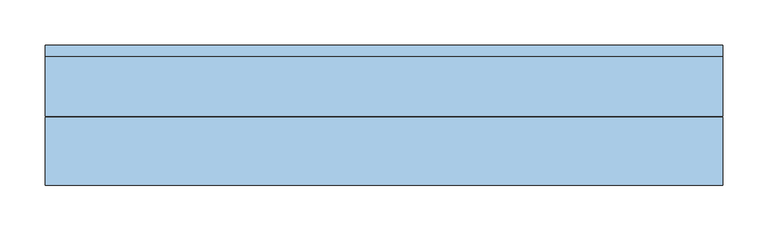
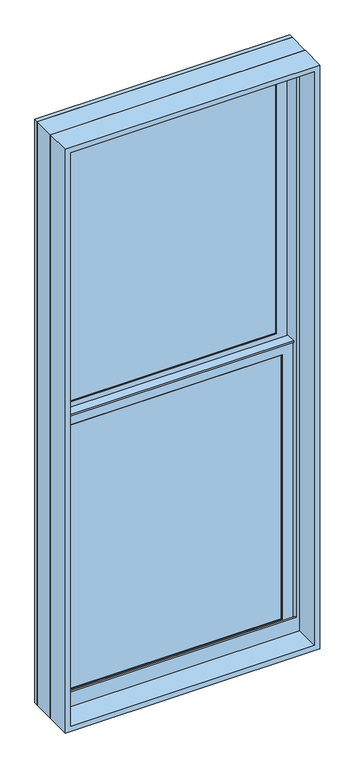
"""IFC4 building model written with IfcOpenShell, lengths in millimetres: window geometry, Window-Double_Hung-Marvin-Essential : ESDH2660."""

import ifcopenshell
import ifcopenshell.guid

model = None  # the IFC model being written
_history = None  # IfcOwnerHistory: only IFC2X3 demands one
_inside = {}  # id of a spatial element -> (the spatial element, [elements in it])
_under = {}  # id of a project, library or spatial element -> (it, [spatial elements below it])
_declared = {}  # id of a project -> (the project, [libraries it declares])
_typed = {}  # id of a type object -> (the type object, [elements of that type])
_made_of = {}  # id of a material, layer set ... -> (it, [elements and type objects made of it])


def new_model(schema):
    """Start an empty IFC model of exactly this schema.

    Asked for "IFC4X3", IfcOpenShell would pick the latest addendum, in which some entities
    have other attributes; the version numbers below select the first issue.
    IFC2X3 requires an IfcOwnerHistory on every rooted entity: one is made here for all.
    """
    global model, _history
    if schema == "IFC4X3":
        model = ifcopenshell.file(schema_version=(4, 3, 0, 0))
    else:
        model = ifcopenshell.file(schema=schema)
    _inside.clear()
    _under.clear()
    _declared.clear()
    _typed.clear()
    _made_of.clear()
    _history = None
    if model.schema == "IFC2X3":
        org = make("IfcOrganization", Name="unknown")
        user = make(
            "IfcPersonAndOrganization",
            ThePerson=make("IfcPerson", FamilyName="unknown"),
            TheOrganization=org,
        )
        app = make(
            "IfcApplication",
            ApplicationDeveloper=org,
            Version="unknown",
            ApplicationFullName="unknown",
            ApplicationIdentifier="unknown",
        )
        _history = make(
            "IfcOwnerHistory",
            OwningUser=user,
            OwningApplication=app,
            ChangeAction="ADDED",
            CreationDate=0,
        )
    return model


def make(cls, **values):
    """One entity of the class cls with the attributes given. An attribute that is None is left unset."""
    return model.create_entity(
        cls, **{name: value for name, value in values.items() if value is not None}
    )


def rooted(cls, **values):
    """An entity with a GlobalId (a new one), such as an element, a storey or a relation."""
    return make(cls, GlobalId=ifcopenshell.guid.new(), OwnerHistory=_history, **values)


def si_unit(unit_type, name, prefix=None):
    """IfcSIUnit, for example si_unit("LENGTHUNIT", "METRE", prefix="MILLI")."""
    return make("IfcSIUnit", UnitType=unit_type, Prefix=prefix, Name=name)


def assignment(units):
    """IfcUnitAssignment: the units of a project."""
    return None if units is None else make("IfcUnitAssignment", Units=units)


def point(xyz):
    """IfcCartesianPoint."""
    return None if xyz is None else make("IfcCartesianPoint", Coordinates=xyz)


def direction(xyz):
    """IfcDirection."""
    return None if xyz is None else make("IfcDirection", DirectionRatios=xyz)


def frame(location, z_axis=None, x_axis=None):
    """IfcAxis2Placement3D, a coordinate frame: its origin and axes. An axis left out is left unset."""
    return make(
        "IfcAxis2Placement3D",
        Location=point(location),
        Axis=direction(z_axis),
        RefDirection=direction(x_axis),
    )


def origin():
    """The frame at (0, 0, 0) with its axes left unset."""
    return frame((0.0, 0.0, 0.0))


def place(relative_to, where):
    """IfcLocalPlacement: puts the frame where relative to a parent placement (None: the world)."""
    return make(
        "IfcLocalPlacement", PlacementRelTo=relative_to, RelativePlacement=where
    )


def context(
    kind, dimensions, precision=None, world=None, true_north=None, identifier=None
):
    """IfcGeometricRepresentationContext, for example the 3D "Model" context."""
    return make(
        "IfcGeometricRepresentationContext",
        ContextIdentifier=identifier,
        ContextType=kind,
        CoordinateSpaceDimension=dimensions,
        Precision=precision,
        WorldCoordinateSystem=world,
        TrueNorth=true_north,
    )


def project(units=None, contexts=None):
    """IfcProject with its units and contexts."""
    return rooted(
        "IfcProject",
        Name="project",
        RepresentationContexts=contexts,
        UnitsInContext=assignment(units),
    )


def spatial(cls, under=None, at=None, **own):
    """A site, building, storey or space (cls), placed at a placement, below another one or the project."""
    s = rooted(cls, ObjectPlacement=at, **own)
    if under is not None:
        _under.setdefault(under.id(), (under, []))[1].append(s)
    return s


def polyline(points):
    """IfcPolyline through the points."""
    return make("IfcPolyline", Points=[point(p) for p in points])


def outline(outer, holes=None, kind="AREA"):
    """IfcArbitraryClosedProfileDef: a profile drawn as a closed curve; with holes, ...WithVoids."""
    if holes is None:
        return make("IfcArbitraryClosedProfileDef", ProfileType=kind, OuterCurve=outer)
    return make(
        "IfcArbitraryProfileDefWithVoids",
        ProfileType=kind,
        OuterCurve=outer,
        InnerCurves=holes,
    )


def extrude(swept, where, along, depth):
    """IfcExtrudedAreaSolid: the profile swept, set in the frame where, extruded along a direction by depth."""
    return make(
        "IfcExtrudedAreaSolid",
        SweptArea=swept,
        Position=where,
        ExtrudedDirection=direction(along),
        Depth=depth,
    )


def faces_of(points, faces, orient=None, outer=None):
    """IfcFace entities. A face is a list of loops; a loop is a list of indices into points, from 0.

    orient and outer hold one flag for each loop. By default every Orientation is true, the
    first loop of a face is its IfcFaceOuterBound and the others are IfcFaceBound.
    """
    made = []
    for i, loops in enumerate(faces):
        bounds = []
        for j, loop in enumerate(loops):
            is_outer = j == 0 if outer is None else outer[i][j]
            bounds.append(
                make(
                    "IfcFaceOuterBound" if is_outer else "IfcFaceBound",
                    Bound=make("IfcPolyLoop", Polygon=[points[k] for k in loop]),
                    Orientation=True if orient is None else orient[i][j],
                )
            )
        made.append(make("IfcFace", Bounds=bounds))
    return made


def faceted_brep(points, faces, orient=None, outer=None, voids=None):
    """IfcFacetedBrep: a solid bounded by flat faces; with voids (closed shells), ...WithVoids."""
    shared = [point(p) for p in points]
    hull = make("IfcClosedShell", CfsFaces=faces_of(shared, faces, orient, outer))
    if voids is None:
        return make("IfcFacetedBrep", Outer=hull)
    return make(
        "IfcFacetedBrepWithVoids",
        Outer=hull,
        Voids=[
            make(cls, CfsFaces=faces_of(shared, fs, o, b)) for cls, fs, o, b in voids
        ],
    )


def shape(context_of_items, identifier, shape_type, items):
    """IfcShapeRepresentation: the items that make up one representation, for example the "Body"."""
    return make(
        "IfcShapeRepresentation",
        ContextOfItems=context_of_items,
        RepresentationIdentifier=identifier,
        RepresentationType=shape_type,
        Items=items,
    )


def source(mapping_origin, context_of_items, identifier, shape_type, items):
    """IfcRepresentationMap: a shape defined once, which mapped items show again and again."""
    return make(
        "IfcRepresentationMap",
        MappingOrigin=mapping_origin,
        MappedRepresentation=shape(context_of_items, identifier, shape_type, items),
    )


def transform(
    local_origin,
    x_axis=None,
    y_axis=None,
    z_axis=None,
    scale=None,
    scale2=None,
    scale3=None,
    uniform=True,
):
    """IfcCartesianTransformationOperator3D, or its non-uniform kind. x_axis, y_axis, z_axis: its Axis1, 2, 3."""
    if uniform:
        return make(
            "IfcCartesianTransformationOperator3D",
            Axis1=direction(x_axis),
            Axis2=direction(y_axis),
            LocalOrigin=point(local_origin),
            Scale=scale,
            Axis3=direction(z_axis),
        )
    return make(
        "IfcCartesianTransformationOperator3DnonUniform",
        Axis1=direction(x_axis),
        Axis2=direction(y_axis),
        LocalOrigin=point(local_origin),
        Scale=scale,
        Axis3=direction(z_axis),
        Scale2=scale2,
        Scale3=scale3,
    )


def mapped(mapping_source, mapping_target):
    """IfcMappedItem: shows the shape of a source again, moved by a transform."""
    return make(
        "IfcMappedItem", MappingSource=mapping_source, MappingTarget=mapping_target
    )


def made_of(thing, what):
    """Note that an element or type object is made of a material, layer set ...; save() writes the relation."""
    if what is not None:
        _made_of.setdefault(what.id(), (what, []))[1].append(thing)
    return thing


def element(
    cls,
    number,
    at=None,
    inside=None,
    cuts=None,
    type_object=None,
    material=None,
    context=None,
    identifier="Body",
    shape_type=None,
    held_by="IfcProductDefinitionShape",
    body=None,
    shapes=None,
    **own,
):
    """One element of the class cls, such as IfcWall. Its Tag is "e" and its number.

    at: its placement. inside: the storey or other place that contains it. cuts: it is an
    opening in that element (IfcRelVoidsElement). A single representation is given by context,
    identifier, shape_type and body (its items); several are given by shapes. held_by: the class
    of the entity that holds the representations. save() writes the other relations.
    """
    e = rooted(cls, Tag="e%d" % number, ObjectPlacement=at, **own)
    if body is not None:
        shapes = [shape(context, identifier, shape_type, body)]
    if shapes is not None:
        e.Representation = make(held_by, Representations=shapes)
    if inside is not None:
        _inside.setdefault(inside.id(), (inside, []))[1].append(e)
    if cuts is not None:
        rooted(
            "IfcRelVoidsElement", RelatingBuildingElement=cuts, RelatedOpeningElement=e
        )
    if type_object is not None:
        _typed.setdefault(type_object.id(), (type_object, []))[1].append(e)
    return made_of(e, material)


def aggregate(whole, parts):
    """IfcRelAggregates: a whole, such as a stair, and the parts it consists of."""
    return rooted("IfcRelAggregates", RelatingObject=whole, RelatedObjects=parts)


def save(model, path):
    """Write the relations noted so far, then the file.

    IfcRelAggregates (storeys below a building ...), IfcRelContainedInSpatialStructure (elements
    in a storey), IfcRelDefinesByType, IfcRelAssociatesMaterial and IfcRelDeclares: one each for
    every whole, place, type object, material and project.
    """
    for whole, parts in _under.values():
        aggregate(whole, parts)
    for where, things in _inside.values():
        rooted(
            "IfcRelContainedInSpatialStructure",
            RelatedElements=things,
            RelatingStructure=where,
        )
    for kind, things in _typed.values():
        rooted("IfcRelDefinesByType", RelatedObjects=things, RelatingType=kind)
    for what, things in _made_of.values():
        rooted("IfcRelAssociatesMaterial", RelatedObjects=things, RelatingMaterial=what)
    for by, libraries in _declared.values():
        rooted("IfcRelDeclares", RelatingContext=by, RelatedDefinitions=libraries)
    model.write(path)


def window_e5f0666e(model_context):
    return source(origin(), model_context, "Body", "SolidModel", [
        extrude(outline(polyline([(115.3583333, 20.6375), (115.3583333, 15.875), (96.3083333, 15.875), (96.3083333, 20.6375), (115.3583333, 20.6375)])), frame((0.0, 0.0, 679.45), z_axis=(0.0, 0.0, 1.0), x_axis=(1.0, 0.0, 0.0)), (0.0, 0.0, 1.0), 831.85),
        extrude(outline(polyline([(-96.3083333, 20.6375), (-96.3083333, 15.875), (-115.3583333, 15.875), (-115.3583333, 20.6375), (-96.3083333, 20.6375)])), frame((0.0, 0.0, 679.45), z_axis=(0.0, 0.0, 1.0), x_axis=(1.0, 0.0, 0.0)), (0.0, 0.0, 1.0), 831.85),
        extrude(outline(polyline([(317.5, 20.6375), (317.5, 15.875), (-317.5, 15.875), (-317.5, 20.6375), (317.5, 20.6375)])), frame((0.0, 0.0, 1085.85), z_axis=(0.0, 0.0, 1.0), x_axis=(1.0, 0.0, 0.0)), (0.0, 0.0, 1.0), 19.05),
        extrude(outline(polyline([(-115.3583333, 46.83125), (-115.3583333, 51.59375), (-96.3083333, 51.59375), (-96.3083333, 46.83125), (-115.3583333, 46.83125)])), frame((0.0, 0.0, 1549.4), z_axis=(0.0, 0.0, 1.0), x_axis=(1.0, 0.0, 0.0)), (0.0, 0.0, 1.0), 831.85),
        extrude(outline(polyline([(96.3083333, 46.83125), (96.3083333, 51.59375), (115.3583333, 51.59375), (115.3583333, 46.83125), (96.3083333, 46.83125)])), frame((0.0, 0.0, 1549.4), z_axis=(0.0, 0.0, 1.0), x_axis=(1.0, 0.0, 0.0)), (0.0, 0.0, 1.0), 831.85),
        extrude(outline(polyline([(-317.5, 46.83125), (-317.5, 51.59375), (317.5, 51.59375), (317.5, 46.83125), (-317.5, 46.83125)])), frame((0.0, 0.0, 1955.8), z_axis=(0.0, 0.0, 1.0), x_axis=(1.0, 0.0, 0.0)), (0.0, 0.0, 1.0), 19.05),
        extrude(outline(polyline([(115.3583333, 20.6375), (96.3083333, 20.6375), (96.3083333, 25.4), (115.3583333, 25.4), (115.3583333, 20.6375)])), frame((0.0, 0.0, 679.45), z_axis=(0.0, 0.0, 1.0), x_axis=(1.0, 0.0, 0.0)), (0.0, 0.0, 1.0), 831.85),
        extrude(outline(polyline([(-96.3083333, 20.6375), (-115.3583333, 20.6375), (-115.3583333, 25.4), (-96.3083333, 25.4), (-96.3083333, 20.6375)])), frame((0.0, 0.0, 679.45), z_axis=(0.0, 0.0, 1.0), x_axis=(1.0, 0.0, 0.0)), (0.0, 0.0, 1.0), 831.85),
        extrude(outline(polyline([(317.5, 20.6375), (-317.5, 20.6375), (-317.5, 25.4), (317.5, 25.4), (317.5, 20.6375)])), frame((0.0, 0.0, 1085.85), z_axis=(0.0, 0.0, 1.0), x_axis=(1.0, 0.0, 0.0)), (0.0, 0.0, 1.0), 19.05),
        extrude(outline(polyline([(-115.3583333, 56.35625), (-96.3083333, 56.35625), (-96.3083333, 51.59375), (-115.3583333, 51.59375), (-115.3583333, 56.35625)])), frame((0.0, 0.0, 1549.4), z_axis=(0.0, 0.0, 1.0), x_axis=(1.0, 0.0, 0.0)), (0.0, 0.0, 1.0), 831.85),
        extrude(outline(polyline([(96.3083333, 56.35625), (115.3583333, 56.35625), (115.3583333, 51.59375), (96.3083333, 51.59375), (96.3083333, 56.35625)])), frame((0.0, 0.0, 1549.4), z_axis=(0.0, 0.0, 1.0), x_axis=(1.0, 0.0, 0.0)), (0.0, 0.0, 1.0), 831.85),
        extrude(outline(polyline([(-317.5, 56.35625), (317.5, 56.35625), (317.5, 51.59375), (-317.5, 51.59375), (-317.5, 56.35625)])), frame((0.0, 0.0, 1955.8), z_axis=(0.0, 0.0, 1.0), x_axis=(1.0, 0.0, 0.0)), (0.0, 0.0, 1.0), 19.05),
        faceted_brep([(-344.4875, 5.6780605, 1541.3351748), (-344.4875, 5.6780605, 1536.7), (344.4875, 5.6780605, 1536.7), (344.4875, 5.6780605, 1541.3351748), (-344.4875, 34.8118605, 1541.3351748), (344.4875, 34.8118605, 1541.3351748), (344.4875, 34.8118605, 1536.7), (-344.4875, 34.8118605, 1536.7), (-344.4875, 30.1625, 1536.7), (-344.4875, 30.1625, 652.4625), (-344.4875, 8.9241104, 652.4625), (-344.4875, 8.9241104, 1536.7), (344.4875, 8.9241104, 1536.7), (344.4875, 30.1625, 1536.7), (344.4875, 8.9241104, 652.4625), (344.4875, 30.1625, 652.4625), (-328.6034752, 11.90625, 1522.4034752), (-328.6034752, 30.1625, 1522.4034752), (328.6034752, 30.1625, 1522.4034752), (328.6034752, 11.90625, 1522.4034752), (-311.94375, 10.4662439, 1505.74375), (-311.94375, 11.90625, 1505.74375), (311.94375, 11.90625, 1505.74375), (311.94375, 10.4662439, 1505.74375), (313.4858834, 8.9241104, 1507.2858834), (-313.4858834, 8.9241104, 1507.2858834), (328.6034752, 30.1625, 668.3465248), (328.6034752, 11.90625, 668.3465248), (311.94375, 11.90625, 685.00625), (311.94375, 10.4662439, 685.00625), (313.4858834, 8.9241104, 683.4641166), (-328.6034752, 30.1625, 668.3465248), (-328.6034752, 11.90625, 668.3465248), (-311.94375, 11.90625, 685.00625), (-311.94375, 10.4662439, 685.00625), (-313.4858834, 8.9241104, 683.4641166)], [[[0, 1, 2, 3]], [[4, 5, 6, 7]], [[1, 0, 4, 7, 8, 9, 10, 11]], [[2, 1, 11, 12]], [[7, 6, 13, 8]], [[3, 2, 12, 14, 15, 13, 6, 5]], [[0, 3, 5, 4]], [[16, 17, 18, 19]], [[20, 21, 22, 23]], [[20, 23, 24, 25]], [[19, 18, 26, 27]], [[23, 22, 28, 29]], [[24, 23, 29, 30]], [[27, 26, 31, 32]], [[29, 28, 33, 34]], [[30, 29, 34, 35]], [[15, 14, 10, 9]], [[15, 9, 8, 13], [18, 17, 31, 26]], [[17, 16, 32, 31]], [[16, 19, 27, 32], [22, 21, 33, 28]], [[21, 20, 34, 33]], [[20, 25, 35, 34]], [[10, 14, 12, 11], [25, 24, 30, 35]]]),
        extrude(outline(polyline([(38.5955581, 1522.4125), (33.5778968, 1522.4125), (33.5778968, 1524.0), (39.9405976, 1524.0), (39.9405976, 1522.4125), (61.515625, 1522.4125), (47.6307501, 1519.0975159), (38.5955581, 1519.0975159), (38.5955581, 1522.4125)])), frame((-344.4875, 0.0, 0.0), z_axis=(1.0, 0.0, 0.0), x_axis=(0.0, 1.0, 0.0)), (0.0, 0.0, 1.0), 688.975),
        faceted_brep([(374.65, 0.0, 622.3), (374.65, 0.0, 2438.4), (-374.65, 0.0, 2438.4), (-374.65, 0.0, 622.3), (348.45625, 0.0, 683.41875), (-348.45625, 0.0, 683.41875), (-348.45625, 0.0, 2412.20625), (348.45625, 0.0, 2412.20625), (348.45625, 3.96875, 622.3), (-348.45625, 3.96875, 622.3), (-348.45625, 3.96875, 683.41875), (348.45625, 3.96875, 683.41875), (-374.65, 65.6828125, 622.3), (-348.45625, 65.6828125, 622.3), (348.45625, 65.6828125, 622.3), (374.65, 65.6828125, 622.3), (-374.65, 65.6828125, 2438.4), (374.65, 65.6828125, 2438.4), (348.45625, 65.6828125, 2412.20625), (-348.45625, 65.6828125, 2412.20625)], [[[0, 1, 2, 3], [4, 5, 6, 7]], [[8, 9, 10, 11]], [[5, 4, 11, 10]], [[0, 3, 12, 13, 9, 8, 14, 15]], [[13, 12, 16, 17, 15, 14, 18, 19]], [[13, 19, 6, 5, 10, 9]], [[7, 6, 19, 18]], [[18, 14, 8, 11, 4, 7]], [[1, 0, 15, 17]], [[2, 1, 17, 16]], [[3, 2, 16, 12]]]),
        faceted_brep([(348.45625, 30.1625, 1530.35), (346.86875, 30.1625, 1530.35), (346.86875, 30.1625, 646.6544613), (348.45625, 30.1625, 646.6544613), (-346.86875, 30.1625, 1530.35), (-348.45625, 30.1625, 1530.35), (-348.45625, 30.1625, 646.6544613), (-346.86875, 30.1625, 646.6544613), (346.86875, 63.5, 1530.35), (348.45625, 63.5, 1530.35), (348.45625, 63.5, 640.1743077), (346.86875, 63.5, 640.1743077), (-348.45625, 63.5, 1530.35), (-346.86875, 63.5, 1530.35), (-346.86875, 63.5, 640.1743077), (-348.45625, 63.5, 640.1743077), (359.7108932, 3.96875, 651.7460105), (359.7108932, 3.96875, 622.3), (359.7108932, 65.6828125, 622.3), (359.7108932, 65.6828125, 639.750012), (-359.7108932, 3.96875, 622.3), (-359.7108932, 3.96875, 651.7460105), (-359.7108932, 65.6828125, 639.750012), (-359.7108932, 65.6828125, 622.3), (359.7108932, 78.58125, 637.2428097), (-359.7108932, 78.58125, 637.2428097), (-357.6971252, 68.2348864, 639.2539391), (-339.73135, 68.2348864, 639.2539391), (-339.73135, 65.6828125, 639.750012), (339.73135, 65.6828125, 639.750012), (339.73135, 68.2348864, 639.2539391), (357.6971252, 68.2348864, 639.2539391), (-374.65, 65.6828125, 622.3), (-374.65, 78.5948249, 622.3), (374.65, 78.5948249, 622.3), (374.65, 65.6828125, 622.3), (-374.65, 78.58125, 2438.4), (374.65, 78.58125, 2438.4), (359.7108932, 78.58125, 2423.4608932), (-359.7108932, 78.58125, 2423.4608932), (-374.65, 65.6828125, 2438.4), (-357.6971252, 68.2348864, 2421.4471252), (357.6971252, 68.2348864, 2421.4471252), (339.73135, 68.2348864, 2403.48135), (-339.73135, 68.2348864, 2403.48135), (-339.73135, 65.6828125, 2403.48135), (339.73135, 65.6828125, 2403.48135), (374.65, 65.6828125, 2438.4)], [[[0, 1, 2, 3]], [[4, 5, 6, 7]], [[8, 9, 10, 11]], [[12, 13, 14, 15]], [[1, 8, 11, 2]], [[9, 0, 3, 10]], [[1, 0, 9, 8]], [[5, 4, 13, 12]], [[5, 12, 15, 6]], [[13, 4, 7, 14]], [[16, 17, 18, 19]], [[20, 21, 22, 23]], [[24, 25, 26, 27, 28, 22, 21, 16, 19, 29, 30, 31], [3, 2, 11, 10], [7, 6, 15, 14]], [[17, 16, 21, 20]], [[17, 20, 23, 32, 33, 34, 35, 18]], [[34, 33, 36, 37], [25, 24, 38, 39]], [[33, 32, 40, 36]], [[39, 41, 26, 25]], [[41, 42, 31, 30, 43, 44, 27, 26]], [[44, 45, 28, 27]], [[40, 32, 23, 22, 28, 45, 46, 29, 19, 18, 35, 47]], [[36, 40, 47, 37]], [[39, 38, 42, 41]], [[44, 43, 46, 45]], [[34, 37, 47, 35]], [[42, 38, 24, 31]], [[46, 43, 30, 29]]]),
        extrude(outline(polyline([(324.64375, 11.90625), (-324.64375, 11.90625), (-324.64375, 15.08125), (324.64375, 15.08125), (324.64375, 11.90625)])), frame((0.0, 0.0, 672.30625), z_axis=(0.0, 0.0, 1.0), x_axis=(1.0, 0.0, 0.0)), (0.0, 0.0, 1.0), 846.1375),
        extrude(outline(polyline([(324.64375, 42.8625), (-324.64375, 42.8625), (-324.64375, 46.0375), (324.64375, 46.0375), (324.64375, 42.8625)])), frame((0.0, 0.0, 1542.25625), z_axis=(0.0, 0.0, 1.0), x_axis=(1.0, 0.0, 0.0)), (0.0, 0.0, 1.0), 846.1375),
        faceted_brep([(-311.94375, 31.194477, 1505.74375), (-313.4858834, 32.7366104, 1507.2858834), (313.4858834, 32.7366104, 1507.2858834), (311.94375, 31.194477, 1505.74375), (-311.94375, 30.1625, 1505.74375), (311.94375, 30.1625, 1505.74375), (-344.4875, 32.7366104, 1538.2875), (-344.4875, 30.1625, 1538.2875), (344.4875, 30.1625, 1538.2875), (344.4875, 32.7366104, 1538.2875), (313.4858834, 32.7366104, 683.4641166), (311.94375, 31.194477, 685.00625), (311.94375, 30.1625, 685.00625), (344.4875, 30.1625, 652.4625), (344.4875, 32.7366104, 652.4625), (-313.4858834, 32.7366104, 683.4641166), (-311.94375, 31.194477, 685.00625), (-311.94375, 30.1625, 685.00625), (-344.4875, 30.1625, 652.4625), (-344.4875, 32.7366104, 652.4625)], [[[0, 1, 2, 3]], [[4, 0, 3, 5]], [[6, 7, 8, 9]], [[3, 2, 10, 11]], [[5, 3, 11, 12]], [[9, 8, 13, 14]], [[11, 10, 15, 16]], [[12, 11, 16, 17]], [[14, 13, 18, 19]], [[9, 14, 19, 6], [1, 15, 10, 2]], [[16, 15, 1, 0]], [[17, 16, 0, 4]], [[7, 18, 13, 8], [5, 12, 17, 4]], [[19, 18, 7, 6]]]),
        faceted_brep([(-328.6034752, 42.8625, 2392.3534752), (-328.6034752, 61.11875, 2392.3534752), (328.6034752, 61.11875, 2392.3534752), (328.6034752, 42.8625, 2392.3534752), (-311.94375, 41.4224939, 2375.69375), (-311.94375, 42.8625, 2375.69375), (311.94375, 42.8625, 2375.69375), (311.94375, 41.4224939, 2375.69375), (-313.4858834, 39.8803604, 2377.2358834), (313.4858834, 39.8803604, 2377.2358834), (-344.4875, 61.11875, 2408.2375), (-344.4875, 39.8803604, 2408.2375), (344.4875, 39.8803604, 2408.2375), (344.4875, 61.11875, 2408.2375), (328.6034752, 61.11875, 1538.2965248), (328.6034752, 42.8625, 1538.2965248), (311.94375, 42.8625, 1554.95625), (311.94375, 41.4224939, 1554.95625), (313.4858834, 39.8803604, 1553.4141166), (344.4875, 39.8803604, 1522.4125), (344.4875, 61.11875, 1522.4125), (-328.6034752, 61.11875, 1538.2965248), (-328.6034752, 42.8625, 1538.2965248), (-311.94375, 42.8625, 1554.95625), (-311.94375, 41.4224939, 1554.95625), (-313.4858834, 39.8803604, 1553.4141166), (-344.4875, 39.8803604, 1522.4125), (-344.4875, 61.11875, 1522.4125)], [[[0, 1, 2, 3]], [[4, 5, 6, 7]], [[8, 4, 7, 9]], [[10, 11, 12, 13]], [[3, 2, 14, 15]], [[7, 6, 16, 17]], [[9, 7, 17, 18]], [[13, 12, 19, 20]], [[15, 14, 21, 22]], [[17, 16, 23, 24]], [[18, 17, 24, 25]], [[20, 19, 26, 27]], [[13, 20, 27, 10], [1, 21, 14, 2]], [[22, 21, 1, 0]], [[3, 15, 22, 0], [5, 23, 16, 6]], [[24, 23, 5, 4]], [[25, 24, 4, 8]], [[11, 26, 19, 12], [9, 18, 25, 8]], [[27, 26, 11, 10]]]),
        faceted_brep([(-344.4875, 61.11875, 1522.4125), (-344.4875, 63.6928604, 1522.4125), (344.4875, 63.6928604, 1522.4125), (344.4875, 61.11875, 1522.4125), (-311.94375, 62.150727, 1554.95625), (-311.94375, 61.11875, 1554.95625), (311.94375, 61.11875, 1554.95625), (311.94375, 62.150727, 1554.95625), (-313.4858834, 63.6928604, 1553.4141166), (313.4858834, 63.6928604, 1553.4141166), (344.4875, 63.6928604, 2408.2375), (344.4875, 61.11875, 2408.2375), (311.94375, 61.11875, 2375.69375), (311.94375, 62.150727, 2375.69375), (313.4858834, 63.6928604, 2377.2358834), (-344.4875, 63.6928604, 2408.2375), (-344.4875, 61.11875, 2408.2375), (-311.94375, 61.11875, 2375.69375), (-311.94375, 62.150727, 2375.69375), (-313.4858834, 63.6928604, 2377.2358834)], [[[0, 1, 2, 3]], [[4, 5, 6, 7]], [[8, 4, 7, 9]], [[3, 2, 10, 11]], [[7, 6, 12, 13]], [[9, 7, 13, 14]], [[11, 10, 15, 16]], [[13, 12, 17, 18]], [[14, 13, 18, 19]], [[16, 15, 1, 0]], [[3, 11, 16, 0], [5, 17, 12, 6]], [[18, 17, 5, 4]], [[19, 18, 4, 8]], [[1, 15, 10, 2], [9, 14, 19, 8]]]),
        extrude(outline(polyline([(324.64375, 26.19375), (-324.64375, 26.19375), (-324.64375, 30.1625), (324.64375, 30.1625), (324.64375, 26.19375)])), frame((0.0, 0.0, 672.30625), z_axis=(0.0, 0.0, 1.0), x_axis=(1.0, 0.0, 0.0)), (0.0, 0.0, 1.0), 846.1375),
        extrude(outline(polyline([(324.64375, 57.15), (-324.64375, 57.15), (-324.64375, 61.11875), (324.64375, 61.11875), (324.64375, 57.15)])), frame((0.0, 0.0, 1542.25625), z_axis=(0.0, 0.0, 1.0), x_axis=(1.0, 0.0, 0.0)), (0.0, 0.0, 1.0), 846.1375),
        extrude(outline(polyline([(2438.4, 374.65), (2438.4, -374.65), (622.3, -374.65), (622.3, 374.65), (2438.4, 374.65)]), holes=[polyline([(2422.525, 358.775), (638.175, 358.775), (638.175, -358.775), (2422.525, -358.775), (2422.525, 358.775)])]), frame((0.0, -76.2, 0.0), z_axis=(0.0, 1.0, 0.0), x_axis=(0.0, 0.0, 1.0)), (0.0, 0.0, 1.0), 75.40625),
    ])


if __name__ == "__main__":
    model = new_model("IFC4")
    model_context = context("Model", 3, world=origin())
    ifc_project = project(units=[si_unit("LENGTHUNIT", "METRE", prefix="MILLI")], contexts=[model_context])
    site = spatial("IfcSite", under=ifc_project)
    building = spatial("IfcBuilding", under=site)
    placement = place(None, origin())
    window_shape = window_e5f0666e(model_context)
    element("IfcWindow", 1, ObjectType="Window-Double_Hung-Marvin-Essential : ESDH2660", at=placement, inside=building, context=model_context, shape_type="MappedRepresentation", body=[
        mapped(window_shape, transform((0.0, 0.0, 0.0), x_axis=(1.0, 0.0, 0.0), y_axis=(0.0, 1.0, 0.0), z_axis=(0.0, 0.0, 1.0))),
    ])
    save(model, "model.ifc")

# Revit data of these elements
# Type "Window-Double_Hung-Marvin-Essential : ESDH2660"
#   Type Mark = "77"
#   Window Type = "Essential Double Hung"
#   Product data url = "https://bimobject.com/marvin-windows-and-doors/product/marvin-dhwau"
#   Product Guid = "c4a96547-874c-4385-91dc-a058adc19d98"
#   Frame = "All Ultrex"
#   Egress Window = "Yes"
#   URL = "www.marvin.com"
#   Model = "ESDH2660"
#   Manufacturer = "Marvin Windows and Doors"
#   Label Egress = "EGRESS WDW"
#   Glass Type = "IG Low E II with Argon"
#   Design Pressure = "DP40"
#   Description = "3072 DBHG"
#   Analytic Construction = "<None>"
#   Prairie Corner Width = 0' - 4"
#   Prairie Corner Height = 0' - 4"
#   Egress Width = 2' - 2 9/16"
#   Egress Height = 2' - 7 27/128"
#   Rough Width = 2' - 6"
#   Rough Height = 6' - 0"
#   Nominal Width = 2' - 6"
#   Nominal Height = 6' - 0"
#   Inset to Installation Flange [instance default] = 0' - 1"
#   Height = 5' - 11 1/2"
#   Egress Area = 5.75723 SF
#   Default Head Height = 8' - 0"
#   Width = 2' - 5 1/2"
#   Daylight Area = 11.0233 SF
#   DLO Width = 2' - 0 9/16"
#   DLO Height = 2' - 8 5/16"
#   Muntins Top Sash = yes
#   Lites Wide Top Sash = 3
#   Lites Wide Bottom Sash = 3
#   Lites High Top Sash = 2
#   Lites High Bottom Sash = 2
#   Lite Cut Prairie 9 = no
#   Lite Cut HV Grid = yes
#   Muntins Bottom Sash = yes
#   Label Visibility = no
#   Jamb Extension Visibility = yes
#   Edition number = 1
#   Interior Material = Ultrex-Marvin-Stonewhite
#   Glazing Material = Glass-Marvin-IG Low E II with Argon
#   Cladding Material = Ultrex-Marvin-Pebblegray
#   Wall Closure = (empty or 0)
#   Assembly Code = ""
# Element 1 (IfcWindow, "Window-Double_Hung-Marvin-Essential : ESDH2660")
#   Materials on its faces: "Ultrex-Marvin-Pebblegray", "Ultrex-Marvin-Stonewhite", "Glass-Marvin-IG Low E II with Argon"
# Materials
#   "Ultrex-Marvin-Stonewhite": class "Paint", colour RGB 250 251 245, transparency 0
#   "Glass-Marvin-IG Low E II with Argon": class "Glass", colour RGB 0 128 192, transparency 0.85
#   "Ultrex-Marvin-Pebblegray": class "Paint", colour RGB 189 185 173, transparency 0
